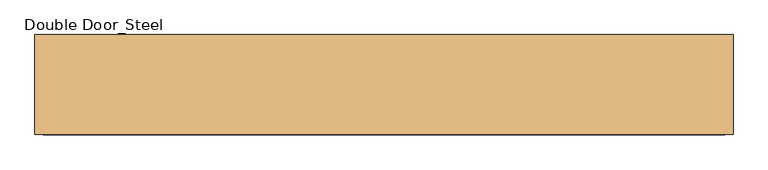
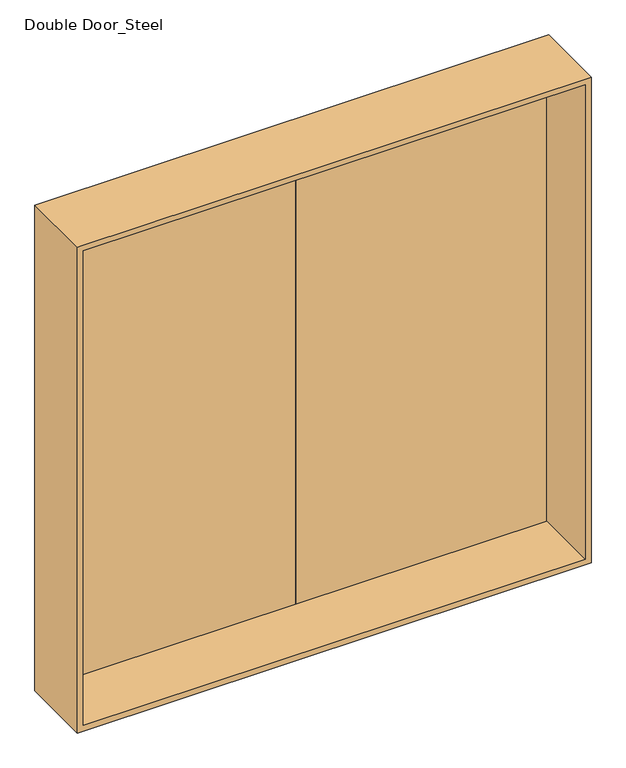
"""IFC4 building model written with IfcOpenShell, lengths in millimetres: door geometry, Double Door_Steel : H_DR_AMB_Double Door_Steel_W3000xH3000."""

import ifcopenshell
import ifcopenshell.guid

model = None  # the IFC model being written
_history = None  # IfcOwnerHistory: only IFC2X3 demands one
_inside = {}  # id of a spatial element -> (the spatial element, [elements in it])
_under = {}  # id of a project, library or spatial element -> (it, [spatial elements below it])
_declared = {}  # id of a project -> (the project, [libraries it declares])
_typed = {}  # id of a type object -> (the type object, [elements of that type])
_made_of = {}  # id of a material, layer set ... -> (it, [elements and type objects made of it])


def new_model(schema):
    """Start an empty IFC model of exactly this schema.

    Asked for "IFC4X3", IfcOpenShell would pick the latest addendum, in which some entities
    have other attributes; the version numbers below select the first issue.
    IFC2X3 requires an IfcOwnerHistory on every rooted entity: one is made here for all.
    """
    global model, _history
    if schema == "IFC4X3":
        model = ifcopenshell.file(schema_version=(4, 3, 0, 0))
    else:
        model = ifcopenshell.file(schema=schema)
    _inside.clear()
    _under.clear()
    _declared.clear()
    _typed.clear()
    _made_of.clear()
    _history = None
    if model.schema == "IFC2X3":
        org = make("IfcOrganization", Name="unknown")
        user = make(
            "IfcPersonAndOrganization",
            ThePerson=make("IfcPerson", FamilyName="unknown"),
            TheOrganization=org,
        )
        app = make(
            "IfcApplication",
            ApplicationDeveloper=org,
            Version="unknown",
            ApplicationFullName="unknown",
            ApplicationIdentifier="unknown",
        )
        _history = make(
            "IfcOwnerHistory",
            OwningUser=user,
            OwningApplication=app,
            ChangeAction="ADDED",
            CreationDate=0,
        )
    return model


def make(cls, **values):
    """One entity of the class cls with the attributes given. An attribute that is None is left unset."""
    return model.create_entity(
        cls, **{name: value for name, value in values.items() if value is not None}
    )


def rooted(cls, **values):
    """An entity with a GlobalId (a new one), such as an element, a storey or a relation."""
    return make(cls, GlobalId=ifcopenshell.guid.new(), OwnerHistory=_history, **values)


def si_unit(unit_type, name, prefix=None):
    """IfcSIUnit, for example si_unit("LENGTHUNIT", "METRE", prefix="MILLI")."""
    return make("IfcSIUnit", UnitType=unit_type, Prefix=prefix, Name=name)


def assignment(units):
    """IfcUnitAssignment: the units of a project."""
    return None if units is None else make("IfcUnitAssignment", Units=units)


def point(xyz):
    """IfcCartesianPoint."""
    return None if xyz is None else make("IfcCartesianPoint", Coordinates=xyz)


def direction(xyz):
    """IfcDirection."""
    return None if xyz is None else make("IfcDirection", DirectionRatios=xyz)


def frame(location, z_axis=None, x_axis=None):
    """IfcAxis2Placement3D, a coordinate frame: its origin and axes. An axis left out is left unset."""
    return make(
        "IfcAxis2Placement3D",
        Location=point(location),
        Axis=direction(z_axis),
        RefDirection=direction(x_axis),
    )


def origin():
    """The frame at (0, 0, 0) with its axes left unset."""
    return frame((0.0, 0.0, 0.0))


def place(relative_to, where):
    """IfcLocalPlacement: puts the frame where relative to a parent placement (None: the world)."""
    return make(
        "IfcLocalPlacement", PlacementRelTo=relative_to, RelativePlacement=where
    )


def context(
    kind, dimensions, precision=None, world=None, true_north=None, identifier=None
):
    """IfcGeometricRepresentationContext, for example the 3D "Model" context."""
    return make(
        "IfcGeometricRepresentationContext",
        ContextIdentifier=identifier,
        ContextType=kind,
        CoordinateSpaceDimension=dimensions,
        Precision=precision,
        WorldCoordinateSystem=world,
        TrueNorth=true_north,
    )


def project(units=None, contexts=None):
    """IfcProject with its units and contexts."""
    return rooted(
        "IfcProject",
        Name="project",
        RepresentationContexts=contexts,
        UnitsInContext=assignment(units),
    )


def spatial(cls, under=None, at=None, **own):
    """A site, building, storey or space (cls), placed at a placement, below another one or the project."""
    s = rooted(cls, ObjectPlacement=at, **own)
    if under is not None:
        _under.setdefault(under.id(), (under, []))[1].append(s)
    return s


def polyline(points):
    """IfcPolyline through the points."""
    return make("IfcPolyline", Points=[point(p) for p in points])


def outline(outer, holes=None, kind="AREA"):
    """IfcArbitraryClosedProfileDef: a profile drawn as a closed curve; with holes, ...WithVoids."""
    if holes is None:
        return make("IfcArbitraryClosedProfileDef", ProfileType=kind, OuterCurve=outer)
    return make(
        "IfcArbitraryProfileDefWithVoids",
        ProfileType=kind,
        OuterCurve=outer,
        InnerCurves=holes,
    )


def extrude(swept, where, along, depth):
    """IfcExtrudedAreaSolid: the profile swept, set in the frame where, extruded along a direction by depth."""
    return make(
        "IfcExtrudedAreaSolid",
        SweptArea=swept,
        Position=where,
        ExtrudedDirection=direction(along),
        Depth=depth,
    )


def faces_of(points, faces, orient=None, outer=None):
    """IfcFace entities. A face is a list of loops; a loop is a list of indices into points, from 0.

    orient and outer hold one flag for each loop. By default every Orientation is true, the
    first loop of a face is its IfcFaceOuterBound and the others are IfcFaceBound.
    """
    made = []
    for i, loops in enumerate(faces):
        bounds = []
        for j, loop in enumerate(loops):
            is_outer = j == 0 if outer is None else outer[i][j]
            bounds.append(
                make(
                    "IfcFaceOuterBound" if is_outer else "IfcFaceBound",
                    Bound=make("IfcPolyLoop", Polygon=[points[k] for k in loop]),
                    Orientation=True if orient is None else orient[i][j],
                )
            )
        made.append(make("IfcFace", Bounds=bounds))
    return made


def faceted_brep(points, faces, orient=None, outer=None, voids=None):
    """IfcFacetedBrep: a solid bounded by flat faces; with voids (closed shells), ...WithVoids."""
    shared = [point(p) for p in points]
    hull = make("IfcClosedShell", CfsFaces=faces_of(shared, faces, orient, outer))
    if voids is None:
        return make("IfcFacetedBrep", Outer=hull)
    return make(
        "IfcFacetedBrepWithVoids",
        Outer=hull,
        Voids=[
            make(cls, CfsFaces=faces_of(shared, fs, o, b)) for cls, fs, o, b in voids
        ],
    )


def shape(context_of_items, identifier, shape_type, items):
    """IfcShapeRepresentation: the items that make up one representation, for example the "Body"."""
    return make(
        "IfcShapeRepresentation",
        ContextOfItems=context_of_items,
        RepresentationIdentifier=identifier,
        RepresentationType=shape_type,
        Items=items,
    )


def source(mapping_origin, context_of_items, identifier, shape_type, items):
    """IfcRepresentationMap: a shape defined once, which mapped items show again and again."""
    return make(
        "IfcRepresentationMap",
        MappingOrigin=mapping_origin,
        MappedRepresentation=shape(context_of_items, identifier, shape_type, items),
    )


def transform(
    local_origin,
    x_axis=None,
    y_axis=None,
    z_axis=None,
    scale=None,
    scale2=None,
    scale3=None,
    uniform=True,
):
    """IfcCartesianTransformationOperator3D, or its non-uniform kind. x_axis, y_axis, z_axis: its Axis1, 2, 3."""
    if uniform:
        return make(
            "IfcCartesianTransformationOperator3D",
            Axis1=direction(x_axis),
            Axis2=direction(y_axis),
            LocalOrigin=point(local_origin),
            Scale=scale,
            Axis3=direction(z_axis),
        )
    return make(
        "IfcCartesianTransformationOperator3DnonUniform",
        Axis1=direction(x_axis),
        Axis2=direction(y_axis),
        LocalOrigin=point(local_origin),
        Scale=scale,
        Axis3=direction(z_axis),
        Scale2=scale2,
        Scale3=scale3,
    )


def mapped(mapping_source, mapping_target):
    """IfcMappedItem: shows the shape of a source again, moved by a transform."""
    return make(
        "IfcMappedItem", MappingSource=mapping_source, MappingTarget=mapping_target
    )


def made_of(thing, what):
    """Note that an element or type object is made of a material, layer set ...; save() writes the relation."""
    if what is not None:
        _made_of.setdefault(what.id(), (what, []))[1].append(thing)
    return thing


def element(
    cls,
    number,
    at=None,
    inside=None,
    cuts=None,
    type_object=None,
    material=None,
    context=None,
    identifier="Body",
    shape_type=None,
    held_by="IfcProductDefinitionShape",
    body=None,
    shapes=None,
    **own,
):
    """One element of the class cls, such as IfcWall. Its Tag is "e" and its number.

    at: its placement. inside: the storey or other place that contains it. cuts: it is an
    opening in that element (IfcRelVoidsElement). A single representation is given by context,
    identifier, shape_type and body (its items); several are given by shapes. held_by: the class
    of the entity that holds the representations. save() writes the other relations.
    """
    e = rooted(cls, Tag="e%d" % number, ObjectPlacement=at, **own)
    if body is not None:
        shapes = [shape(context, identifier, shape_type, body)]
    if shapes is not None:
        e.Representation = make(held_by, Representations=shapes)
    if inside is not None:
        _inside.setdefault(inside.id(), (inside, []))[1].append(e)
    if cuts is not None:
        rooted(
            "IfcRelVoidsElement", RelatingBuildingElement=cuts, RelatedOpeningElement=e
        )
    if type_object is not None:
        _typed.setdefault(type_object.id(), (type_object, []))[1].append(e)
    return made_of(e, material)


def aggregate(whole, parts):
    """IfcRelAggregates: a whole, such as a stair, and the parts it consists of."""
    return rooted("IfcRelAggregates", RelatingObject=whole, RelatedObjects=parts)


def save(model, path):
    """Write the relations noted so far, then the file.

    IfcRelAggregates (storeys below a building ...), IfcRelContainedInSpatialStructure (elements
    in a storey), IfcRelDefinesByType, IfcRelAssociatesMaterial and IfcRelDeclares: one each for
    every whole, place, type object, material and project.
    """
    for whole, parts in _under.values():
        aggregate(whole, parts)
    for where, things in _inside.values():
        rooted(
            "IfcRelContainedInSpatialStructure",
            RelatedElements=things,
            RelatingStructure=where,
        )
    for kind, things in _typed.values():
        rooted("IfcRelDefinesByType", RelatedObjects=things, RelatingType=kind)
    for what, things in _made_of.values():
        rooted("IfcRelAssociatesMaterial", RelatedObjects=things, RelatingMaterial=what)
    for by, libraries in _declared.values():
        rooted("IfcRelDeclares", RelatingContext=by, RelatedDefinitions=libraries)
    model.write(path)


def double_door_steel_89dfd0fe(model_context):
    return source(origin(), model_context, "Body", "SolidModel", [
        extrude(outline(polyline([(1480.0, 175.0), (0.0, 175.0), (0.0, 215.0), (1480.0, 215.0), (1480.0, 175.0)])), frame((0.0, 0.0, 20.0), z_axis=(0.0, 0.0, 1.0), x_axis=(1.0, 0.0, 0.0)), (0.0, 0.0, 1.0), 2960.0),
        extrude(outline(polyline([(0.0, 175.0), (-1480.0, 175.0), (-1480.0, 215.0), (0.0, 215.0), (0.0, 175.0)])), frame((0.0, 0.0, 20.0), z_axis=(0.0, 0.0, 1.0), x_axis=(1.0, 0.0, 0.0)), (0.0, 0.0, 1.0), 2960.0),
        faceted_brep([(1500.0, -215.0, 3000.0), (1500.0, 215.0, 3000.0), (-1500.0, 215.0, 3000.0), (-1500.0, -215.0, 3000.0), (1465.0, 175.0, 2965.0), (1465.0, -215.0, 2965.0), (-1465.0, -215.0, 2965.0), (-1465.0, 175.0, 2965.0), (1480.0, 215.0, 2980.0), (1480.0, 175.0, 2980.0), (-1480.0, 175.0, 2980.0), (-1480.0, 215.0, 2980.0), (-1500.0, 215.0, 0.0), (-1500.0, -215.0, 0.0), (-1465.0, -215.0, 35.0), (-1465.0, 175.0, 35.0), (-1480.0, 175.0, 20.0), (-1480.0, 215.0, 20.0), (1500.0, 215.0, 0.0), (1480.0, 215.0, 20.0), (1500.0, -215.0, 0.0), (1465.0, -215.0, 35.0), (1465.0, 175.0, 35.0), (1480.0, 175.0, 20.0)], [[[0, 1, 2, 3]], [[4, 5, 6, 7]], [[8, 9, 10, 11]], [[3, 2, 12, 13]], [[7, 6, 14, 15]], [[11, 10, 16, 17]], [[18, 12, 2, 1], [8, 11, 17, 19]], [[13, 12, 18, 20]], [[0, 3, 13, 20], [21, 14, 6, 5]], [[15, 14, 21, 22]], [[23, 16, 10, 9], [4, 7, 15, 22]], [[17, 16, 23, 19]], [[20, 18, 1, 0]], [[22, 21, 5, 4]], [[19, 23, 9, 8]]]),
    ])


if __name__ == "__main__":
    model = new_model("IFC4")
    model_context = context("Model", 3, world=origin())
    ifc_project = project(units=[si_unit("LENGTHUNIT", "METRE", prefix="MILLI")], contexts=[model_context])
    site = spatial("IfcSite", under=ifc_project)
    building = spatial("IfcBuilding", under=site)
    placement = place(None, origin())
    double_door_steel_shape = double_door_steel_89dfd0fe(model_context)
    element("IfcDoor", 1, ObjectType="Double Door_Steel : H_DR_AMB_Double Door_Steel_W3000xH3000", at=placement, inside=building, context=model_context, shape_type="MappedRepresentation", body=[
        mapped(double_door_steel_shape, transform((0.0, 0.0, 0.0), x_axis=(1.0, 0.0, 0.0), y_axis=(0.0, 1.0, 0.0), z_axis=(0.0, 0.0, 1.0))),
    ])
    save(model, "model.ifc")

# Revit data of these elements
# Type "Double Door_Steel : H_DR_AMB_Double Door_Steel_W3000xH3000"
#   Type Mark = "362"
#   프레임 = ""
#   철물 = ""
#   유리/마감 = ""
#   위치/개소 = ""
#   부호 = "1/SD"
#   문번호 = ""
#   문기호 = "SD"
#   Analytic Construction = "<None>"
#   Height = 3000.000 mm
#   Width = 3000.000 mm
#   Define Thermal Properties by = 1
#   문 틀 = none
#   문 = none
#   Function = (empty or 0)
#   Assembly Code = ""
#   Wall Closure = (empty or 0)
